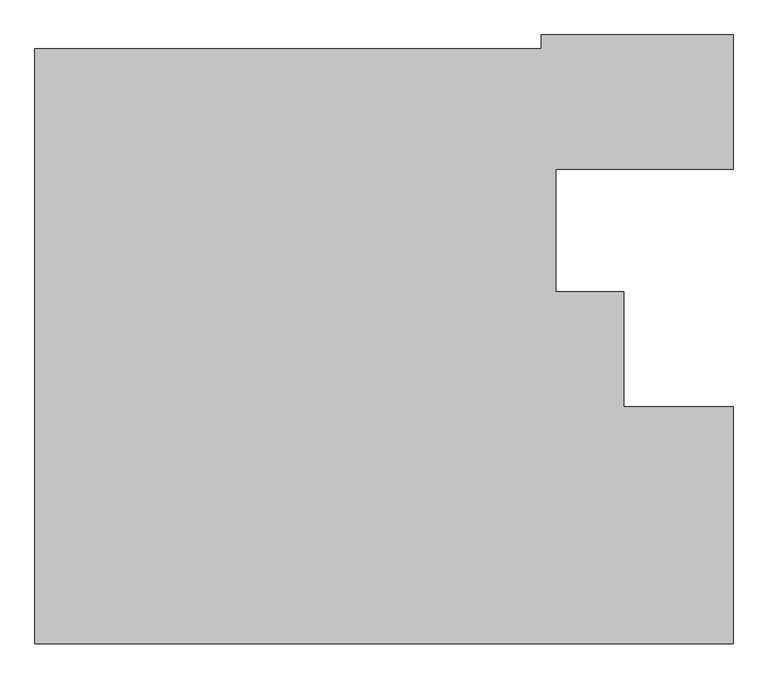
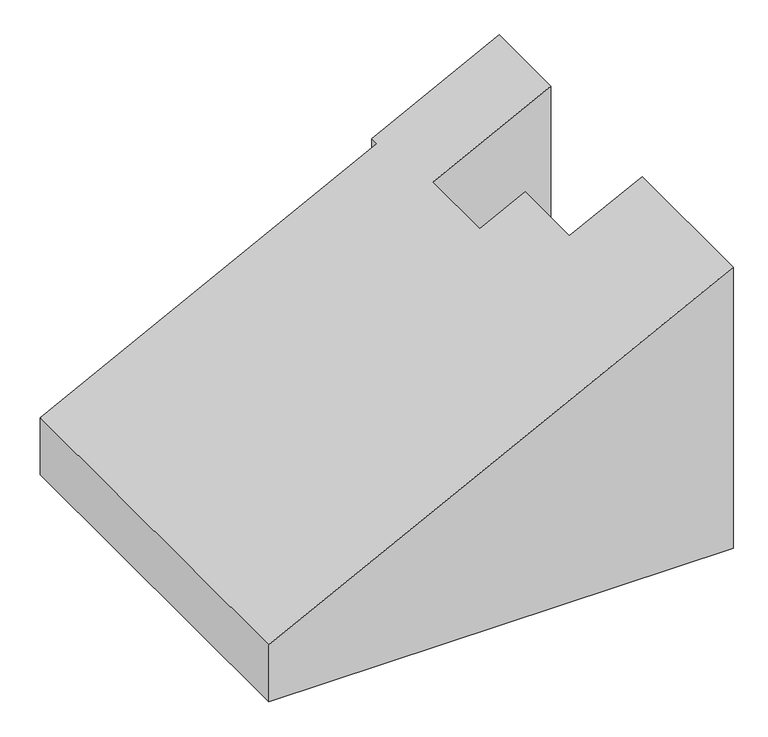
"""IFC4 building model written with IfcOpenShell, lengths in millimetres: proxy geometry, 0_3d."""

import ifcopenshell
import ifcopenshell.guid

model = None  # the IFC model being written
_history = None  # IfcOwnerHistory: only IFC2X3 demands one
_inside = {}  # id of a spatial element -> (the spatial element, [elements in it])
_under = {}  # id of a project, library or spatial element -> (it, [spatial elements below it])
_declared = {}  # id of a project -> (the project, [libraries it declares])
_typed = {}  # id of a type object -> (the type object, [elements of that type])
_made_of = {}  # id of a material, layer set ... -> (it, [elements and type objects made of it])


def new_model(schema):
    """Start an empty IFC model of exactly this schema.

    Asked for "IFC4X3", IfcOpenShell would pick the latest addendum, in which some entities
    have other attributes; the version numbers below select the first issue.
    IFC2X3 requires an IfcOwnerHistory on every rooted entity: one is made here for all.
    """
    global model, _history
    if schema == "IFC4X3":
        model = ifcopenshell.file(schema_version=(4, 3, 0, 0))
    else:
        model = ifcopenshell.file(schema=schema)
    _inside.clear()
    _under.clear()
    _declared.clear()
    _typed.clear()
    _made_of.clear()
    _history = None
    if model.schema == "IFC2X3":
        org = make("IfcOrganization", Name="unknown")
        user = make(
            "IfcPersonAndOrganization",
            ThePerson=make("IfcPerson", FamilyName="unknown"),
            TheOrganization=org,
        )
        app = make(
            "IfcApplication",
            ApplicationDeveloper=org,
            Version="unknown",
            ApplicationFullName="unknown",
            ApplicationIdentifier="unknown",
        )
        _history = make(
            "IfcOwnerHistory",
            OwningUser=user,
            OwningApplication=app,
            ChangeAction="ADDED",
            CreationDate=0,
        )
    return model


def make(cls, **values):
    """One entity of the class cls with the attributes given. An attribute that is None is left unset."""
    return model.create_entity(
        cls, **{name: value for name, value in values.items() if value is not None}
    )


def rooted(cls, **values):
    """An entity with a GlobalId (a new one), such as an element, a storey or a relation."""
    return make(cls, GlobalId=ifcopenshell.guid.new(), OwnerHistory=_history, **values)


def si_unit(unit_type, name, prefix=None):
    """IfcSIUnit, for example si_unit("LENGTHUNIT", "METRE", prefix="MILLI")."""
    return make("IfcSIUnit", UnitType=unit_type, Prefix=prefix, Name=name)


def assignment(units):
    """IfcUnitAssignment: the units of a project."""
    return None if units is None else make("IfcUnitAssignment", Units=units)


def point(xyz):
    """IfcCartesianPoint."""
    return None if xyz is None else make("IfcCartesianPoint", Coordinates=xyz)


def direction(xyz):
    """IfcDirection."""
    return None if xyz is None else make("IfcDirection", DirectionRatios=xyz)


def frame(location, z_axis=None, x_axis=None):
    """IfcAxis2Placement3D, a coordinate frame: its origin and axes. An axis left out is left unset."""
    return make(
        "IfcAxis2Placement3D",
        Location=point(location),
        Axis=direction(z_axis),
        RefDirection=direction(x_axis),
    )


def origin():
    """The frame at (0, 0, 0) with its axes left unset."""
    return frame((0.0, 0.0, 0.0))


def place(relative_to, where):
    """IfcLocalPlacement: puts the frame where relative to a parent placement (None: the world)."""
    return make(
        "IfcLocalPlacement", PlacementRelTo=relative_to, RelativePlacement=where
    )


def context(
    kind, dimensions, precision=None, world=None, true_north=None, identifier=None
):
    """IfcGeometricRepresentationContext, for example the 3D "Model" context."""
    return make(
        "IfcGeometricRepresentationContext",
        ContextIdentifier=identifier,
        ContextType=kind,
        CoordinateSpaceDimension=dimensions,
        Precision=precision,
        WorldCoordinateSystem=world,
        TrueNorth=true_north,
    )


def project(units=None, contexts=None):
    """IfcProject with its units and contexts."""
    return rooted(
        "IfcProject",
        Name="project",
        RepresentationContexts=contexts,
        UnitsInContext=assignment(units),
    )


def spatial(cls, under=None, at=None, **own):
    """A site, building, storey or space (cls), placed at a placement, below another one or the project."""
    s = rooted(cls, ObjectPlacement=at, **own)
    if under is not None:
        _under.setdefault(under.id(), (under, []))[1].append(s)
    return s


def faces_of(points, faces, orient=None, outer=None):
    """IfcFace entities. A face is a list of loops; a loop is a list of indices into points, from 0.

    orient and outer hold one flag for each loop. By default every Orientation is true, the
    first loop of a face is its IfcFaceOuterBound and the others are IfcFaceBound.
    """
    made = []
    for i, loops in enumerate(faces):
        bounds = []
        for j, loop in enumerate(loops):
            is_outer = j == 0 if outer is None else outer[i][j]
            bounds.append(
                make(
                    "IfcFaceOuterBound" if is_outer else "IfcFaceBound",
                    Bound=make("IfcPolyLoop", Polygon=[points[k] for k in loop]),
                    Orientation=True if orient is None else orient[i][j],
                )
            )
        made.append(make("IfcFace", Bounds=bounds))
    return made


def faceted_brep(points, faces, orient=None, outer=None, voids=None):
    """IfcFacetedBrep: a solid bounded by flat faces; with voids (closed shells), ...WithVoids."""
    shared = [point(p) for p in points]
    hull = make("IfcClosedShell", CfsFaces=faces_of(shared, faces, orient, outer))
    if voids is None:
        return make("IfcFacetedBrep", Outer=hull)
    return make(
        "IfcFacetedBrepWithVoids",
        Outer=hull,
        Voids=[
            make(cls, CfsFaces=faces_of(shared, fs, o, b)) for cls, fs, o, b in voids
        ],
    )


def shape(context_of_items, identifier, shape_type, items):
    """IfcShapeRepresentation: the items that make up one representation, for example the "Body"."""
    return make(
        "IfcShapeRepresentation",
        ContextOfItems=context_of_items,
        RepresentationIdentifier=identifier,
        RepresentationType=shape_type,
        Items=items,
    )


def source(mapping_origin, context_of_items, identifier, shape_type, items):
    """IfcRepresentationMap: a shape defined once, which mapped items show again and again."""
    return make(
        "IfcRepresentationMap",
        MappingOrigin=mapping_origin,
        MappedRepresentation=shape(context_of_items, identifier, shape_type, items),
    )


def transform(
    local_origin,
    x_axis=None,
    y_axis=None,
    z_axis=None,
    scale=None,
    scale2=None,
    scale3=None,
    uniform=True,
):
    """IfcCartesianTransformationOperator3D, or its non-uniform kind. x_axis, y_axis, z_axis: its Axis1, 2, 3."""
    if uniform:
        return make(
            "IfcCartesianTransformationOperator3D",
            Axis1=direction(x_axis),
            Axis2=direction(y_axis),
            LocalOrigin=point(local_origin),
            Scale=scale,
            Axis3=direction(z_axis),
        )
    return make(
        "IfcCartesianTransformationOperator3DnonUniform",
        Axis1=direction(x_axis),
        Axis2=direction(y_axis),
        LocalOrigin=point(local_origin),
        Scale=scale,
        Axis3=direction(z_axis),
        Scale2=scale2,
        Scale3=scale3,
    )


def mapped(mapping_source, mapping_target):
    """IfcMappedItem: shows the shape of a source again, moved by a transform."""
    return make(
        "IfcMappedItem", MappingSource=mapping_source, MappingTarget=mapping_target
    )


def made_of(thing, what):
    """Note that an element or type object is made of a material, layer set ...; save() writes the relation."""
    if what is not None:
        _made_of.setdefault(what.id(), (what, []))[1].append(thing)
    return thing


def element(
    cls,
    number,
    at=None,
    inside=None,
    cuts=None,
    type_object=None,
    material=None,
    context=None,
    identifier="Body",
    shape_type=None,
    held_by="IfcProductDefinitionShape",
    body=None,
    shapes=None,
    **own,
):
    """One element of the class cls, such as IfcWall. Its Tag is "e" and its number.

    at: its placement. inside: the storey or other place that contains it. cuts: it is an
    opening in that element (IfcRelVoidsElement). A single representation is given by context,
    identifier, shape_type and body (its items); several are given by shapes. held_by: the class
    of the entity that holds the representations. save() writes the other relations.
    """
    e = rooted(cls, Tag="e%d" % number, ObjectPlacement=at, **own)
    if body is not None:
        shapes = [shape(context, identifier, shape_type, body)]
    if shapes is not None:
        e.Representation = make(held_by, Representations=shapes)
    if inside is not None:
        _inside.setdefault(inside.id(), (inside, []))[1].append(e)
    if cuts is not None:
        rooted(
            "IfcRelVoidsElement", RelatingBuildingElement=cuts, RelatedOpeningElement=e
        )
    if type_object is not None:
        _typed.setdefault(type_object.id(), (type_object, []))[1].append(e)
    return made_of(e, material)


def aggregate(whole, parts):
    """IfcRelAggregates: a whole, such as a stair, and the parts it consists of."""
    return rooted("IfcRelAggregates", RelatingObject=whole, RelatedObjects=parts)


def save(model, path):
    """Write the relations noted so far, then the file.

    IfcRelAggregates (storeys below a building ...), IfcRelContainedInSpatialStructure (elements
    in a storey), IfcRelDefinesByType, IfcRelAssociatesMaterial and IfcRelDeclares: one each for
    every whole, place, type object, material and project.
    """
    for whole, parts in _under.values():
        aggregate(whole, parts)
    for where, things in _inside.values():
        rooted(
            "IfcRelContainedInSpatialStructure",
            RelatedElements=things,
            RelatingStructure=where,
        )
    for kind, things in _typed.values():
        rooted("IfcRelDefinesByType", RelatedObjects=things, RelatingType=kind)
    for what, things in _made_of.values():
        rooted("IfcRelAssociatesMaterial", RelatedObjects=things, RelatingMaterial=what)
    for by, libraries in _declared.values():
        rooted("IfcRelDeclares", RelatingContext=by, RelatedDefinitions=libraries)
    model.write(path)


def generic_models_82b4d27e(model_context):
    return source(origin(), model_context, "Body", "Brep", [
        faceted_brep([(4750.0, 5582.8619019, 3273.5797924), (0.0, 5582.8619019, 853.3339073), (0.0, 0.0, 853.3339073), (6550.0, 0.0, 4190.7256015), (6550.0, 2223.2600653, 4190.7256015), (5525.0, 2223.2600653, 3668.4620158), (5525.0, 3302.8619019, 3668.4620158), (4885.0, 3302.8619019, 3342.3657281), (4885.0, 4452.8619019, 3342.3657281), (6550.0, 4452.8619019, 4190.7256015), (6550.0, 5712.8619019, 4190.7256015), (4750.0, 5712.8619019, 3273.5797924), (5525.0, 3302.8619019, 0.0), (4885.0, 3302.8619019, 0.0), (5525.0, 2223.2600653, 0.0), (6550.0, 2223.2600653, 0.0), (0.0, 0.0, 0.0), (6550.0, 0.0, 0.0), (0.0, 5582.8619019, 0.0), (4750.0, 5582.8619019, 0.0), (4750.0, 5712.8619019, 0.0), (6550.0, 5712.8619019, 0.0), (6550.0, 4452.8619019, 0.0), (4885.0, 4452.8619019, 0.0)], [[[0, 1, 2, 3, 4, 5, 6, 7, 8, 9, 10, 11]], [[7, 6, 12, 13]], [[6, 5, 14, 12]], [[5, 4, 15, 14]], [[3, 2, 16, 17]], [[2, 1, 18, 16]], [[1, 0, 19, 18]], [[0, 11, 20, 19]], [[11, 10, 21, 20]], [[22, 21, 10, 9]], [[9, 8, 23, 22]], [[8, 7, 13, 23]], [[17, 15, 4, 3]], [[16, 18, 19, 20, 21, 22, 23, 13, 12, 14, 15, 17]]]),
    ])


if __name__ == "__main__":
    model = new_model("IFC4")
    model_context = context("Model", 3, world=origin())
    ifc_project = project(units=[si_unit("LENGTHUNIT", "METRE", prefix="MILLI")], contexts=[model_context])
    site = spatial("IfcSite", under=ifc_project)
    building = spatial("IfcBuilding", under=site)
    placement = place(None, origin())
    generic_models_shape = generic_models_82b4d27e(model_context)
    element("IfcBuildingElementProxy", 1, Name="0_3d", ObjectType="0_3d", at=placement, inside=building, context=model_context, shape_type="MappedRepresentation", body=[
        mapped(generic_models_shape, transform((0.0, 0.0, 0.0), x_axis=(1.0, 0.0, 0.0), y_axis=(0.0, 1.0, 0.0), z_axis=(0.0, 0.0, 1.0))),
    ])
    save(model, "model.ifc")

# Revit data of these elements
# Element 1 (IfcBuildingElementProxy, "0_3d")
#   Materials on its faces: "*1"
# Materials
#   "*1": class "Unassigned", colour RGB 175 175 175, transparency 0
